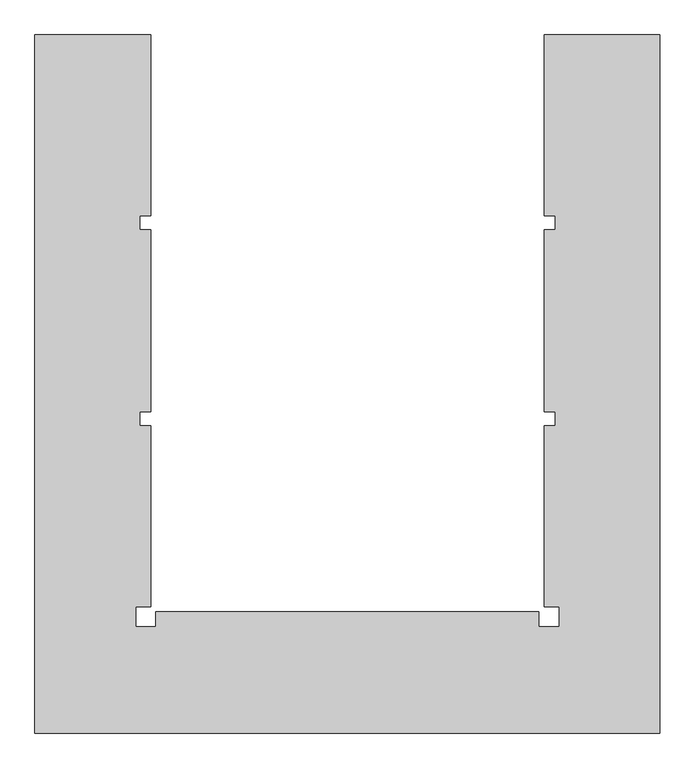
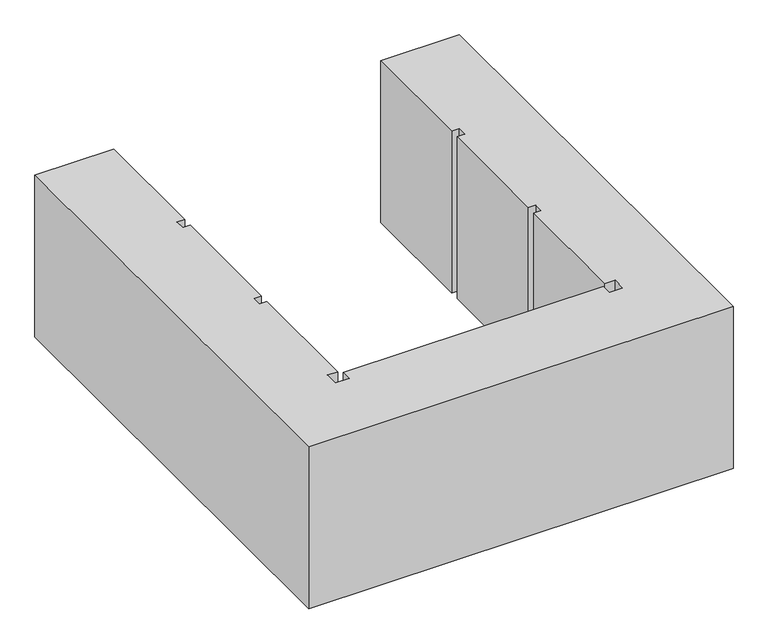
"""IFC4 building model written with IfcOpenShell, lengths in millimetres: proxy geometry, 0_3d."""

from ifc_helpers import new_model, si_unit, origin, origin_with_axes, place, context, project, spatial, polyline, outline, extrude, source, transform, mapped, element, save


def generic_models_1b72f00f(model_context):
    return source(origin(), model_context, "Body", "SweptSolid", [
        extrude(outline(polyline([(0.0, 6925.0), (1150.0, 6925.0), (1150.0, 5131.6), (1040.0, 5131.6), (1040.0, 4991.6), (1150.0, 4991.6), (1150.0, 3188.3), (1040.0, 3188.3), (1040.0, 3048.3), (1150.0, 3048.3), (1150.0, 1255.0), (1000.0, 1255.0), (1000.0, 1055.0), (1200.0, 1055.0), (1200.0, 1205.0), (5000.0, 1205.0), (5000.0, 1055.0), (5200.0, 1055.0), (5200.0, 1255.0), (5050.0, 1255.0), (5050.0, 3048.3), (5160.0, 3048.3), (5160.0, 3188.3), (5050.0, 3188.3), (5050.0, 4991.6), (5160.0, 4991.6), (5160.0, 5131.6), (5050.0, 5131.6), (5050.0, 6925.0), (6200.0, 6925.0), (6200.0, 0.0), (0.0, 0.0), (0.0, 6925.0)])), origin_with_axes(), (0.0, 0.0, 1.0), 2500.0),
    ])


if __name__ == "__main__":
    model = new_model("IFC4")
    model_context = context("Model", 3, world=origin())
    ifc_project = project(units=[si_unit("LENGTHUNIT", "METRE", prefix="MILLI")], contexts=[model_context])
    site = spatial("IfcSite", under=ifc_project)
    building = spatial("IfcBuilding", under=site)
    placement = place(None, origin())
    generic_models_shape = generic_models_1b72f00f(model_context)
    element("IfcBuildingElementProxy", 1, Name="0_3d", ObjectType="0_3d", at=placement, inside=building, context=model_context, shape_type="MappedRepresentation", body=[
        mapped(generic_models_shape, transform((0.0, 0.0, 0.0), x_axis=(1.0, 0.0, 0.0), y_axis=(0.0, 1.0, 0.0), z_axis=(0.0, 0.0, 1.0))),
    ])
    save(model, "model.ifc")

# Revit data of these elements
# Element 1 (IfcBuildingElementProxy, "0_3d")
#   Materials on its faces: "*1"
# Materials
#   "*1": class "Unassigned", colour RGB 175 175 175, transparency 0
